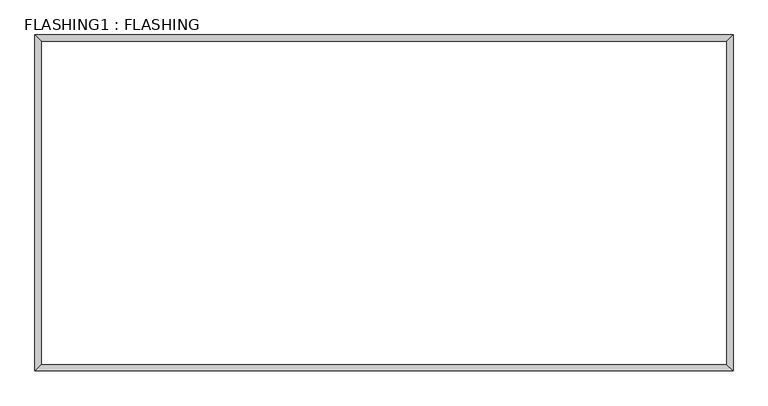
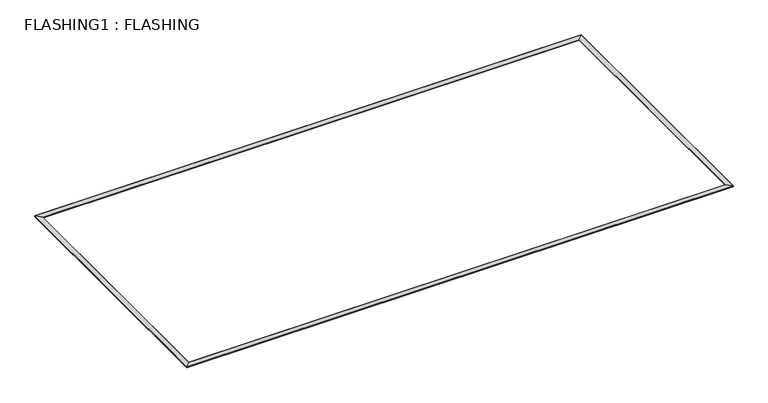
"""IFC4 building model written with IfcOpenShell, lengths in millimetres: proxy geometry, FLASHING1 : FLASHING."""

from ifc_helpers import new_model, si_unit, origin, place, context, project, spatial, faceted_brep, source, transform, mapped, element, save


def flashing1_flashing_4cce81cf(model_context):
    return source(origin(), model_context, "Body", "Brep", [
        faceted_brep([(40720.0, 40009.5208589, 18739.9720055), (40720.0, 40009.5208589, 18724.9720055), (40720.0, 19989.5208589, 18724.9720055), (40720.0, 19989.5208589, 18739.9720055), (40721.0, 40010.5208589, 18750.9720055), (40721.0, 40010.5208589, 18739.9720055), (40721.0, 19988.5208589, 18739.9720055), (40721.0, 19988.5208589, 18750.9720055), (40749.0, 40038.5208589, 18819.1280996), (40749.0, 40038.5208589, 18750.9720055), (40749.0, 19960.5208589, 18750.9720055), (40749.0, 19960.5208589, 18819.1280996), (40371.0, 39660.5208589, 18804.3045702), (40371.0, 20338.5208589, 18804.3045702), (40371.0, 39660.5208589, 18750.9720055), (40371.0, 20338.5208589, 18750.9720055), (40399.0, 39688.5208589, 18739.9720055), (40399.0, 39688.5208589, 18750.9720055), (40399.0, 20310.5208589, 18750.9720055), (40399.0, 20310.5208589, 18739.9720055), (40400.0, 39689.5208589, 18724.9720055), (40400.0, 39689.5208589, 18739.9720055), (40400.0, 20309.5208589, 18739.9720055), (40400.0, 20309.5208589, 18724.9720055), (40398.0, 39687.5208589, 18749.9720055), (40398.0, 39687.5208589, 18724.9720055), (40398.0, 20311.5208589, 18724.9720055), (40398.0, 20311.5208589, 18749.9720055), (40370.0, 39659.5208589, 18805.2661232), (40370.0, 39659.5208589, 18749.9720055), (40370.0, 20339.5208589, 18749.9720055), (40370.0, 20339.5208589, 18805.2661232), (40750.0, 40039.5208589, 18820.168084), (40750.0, 19959.5208589, 18820.168084), (40750.0, 40039.5208589, 18749.9720055), (40750.0, 19959.5208589, 18749.9720055), (40722.0, 40011.5208589, 18724.9720055), (40722.0, 40011.5208589, 18749.9720055), (40722.0, 19987.5208589, 18749.9720055), (40722.0, 19987.5208589, 18724.9720055), (-935.0, 19989.5208589, 18724.9720055), (-935.0, 19989.5208589, 18739.9720055), (-936.0, 19988.5208589, 18739.9720055), (-936.0, 19988.5208589, 18750.9720055), (-964.0, 19960.5208589, 18750.9720055), (-964.0, 19960.5208589, 18819.1280996), (-586.0, 20338.5208589, 18804.3045702), (-586.0, 20338.5208589, 18750.9720055), (-614.0, 20310.5208589, 18750.9720055), (-614.0, 20310.5208589, 18739.9720055), (-615.0, 20309.5208589, 18739.9720055), (-615.0, 20309.5208589, 18724.9720055), (-613.0, 20311.5208589, 18724.9720055), (-613.0, 20311.5208589, 18749.9720055), (-585.0, 20339.5208589, 18749.9720055), (-585.0, 20339.5208589, 18805.2661232), (-965.0, 19959.5208589, 18820.168084), (-965.0, 19959.5208589, 18749.9720055), (-937.0, 19987.5208589, 18749.9720055), (-937.0, 19987.5208589, 18724.9720055), (-935.0, 40009.5208589, 18724.9720055), (-935.0, 40009.5208589, 18739.9720055), (-936.0, 40010.5208589, 18739.9720055), (-936.0, 40010.5208589, 18750.9720055), (-964.0, 40038.5208589, 18750.9720055), (-964.0, 40038.5208589, 18819.1280996), (-586.0, 39660.5208589, 18804.3045702), (-586.0, 39660.5208589, 18750.9720055), (-614.0, 39688.5208589, 18750.9720055), (-614.0, 39688.5208589, 18739.9720055), (-615.0, 39689.5208589, 18739.9720055), (-615.0, 39689.5208589, 18724.9720055), (-613.0, 39687.5208589, 18724.9720055), (-613.0, 39687.5208589, 18749.9720055), (-585.0, 39659.5208589, 18749.9720055), (-585.0, 39659.5208589, 18805.2661232), (-965.0, 40039.5208589, 18820.168084), (-965.0, 40039.5208589, 18749.9720055), (-937.0, 40011.5208589, 18749.9720055), (-937.0, 40011.5208589, 18724.9720055)], [[[0, 1, 2, 3]], [[4, 5, 6, 7]], [[8, 9, 10, 11]], [[12, 8, 11, 13]], [[14, 12, 13, 15]], [[16, 17, 18, 19]], [[20, 21, 22, 23]], [[24, 25, 26, 27]], [[28, 29, 30, 31]], [[32, 28, 31, 33]], [[34, 32, 33, 35]], [[36, 37, 38, 39]], [[3, 2, 40, 41]], [[7, 6, 42, 43]], [[11, 10, 44, 45]], [[13, 11, 45, 46]], [[15, 13, 46, 47]], [[19, 18, 48, 49]], [[23, 22, 50, 51]], [[27, 26, 52, 53]], [[31, 30, 54, 55]], [[33, 31, 55, 56]], [[35, 33, 56, 57]], [[39, 38, 58, 59]], [[41, 40, 60, 61]], [[43, 42, 62, 63]], [[45, 44, 64, 65]], [[46, 45, 65, 66]], [[47, 46, 66, 67]], [[49, 48, 68, 69]], [[51, 50, 70, 71]], [[53, 52, 72, 73]], [[55, 54, 74, 75]], [[56, 55, 75, 76]], [[57, 56, 76, 77]], [[59, 58, 78, 79]], [[61, 60, 1, 0]], [[5, 62, 42, 6], [3, 41, 61, 0]], [[63, 62, 5, 4]], [[9, 64, 44, 10], [7, 43, 63, 4]], [[65, 64, 9, 8]], [[66, 65, 8, 12]], [[67, 66, 12, 14]], [[17, 68, 48, 18], [15, 47, 67, 14]], [[69, 68, 17, 16]], [[21, 70, 50, 22], [19, 49, 69, 16]], [[71, 70, 21, 20]], [[23, 51, 71, 20], [25, 72, 52, 26]], [[73, 72, 25, 24]], [[27, 53, 73, 24], [29, 74, 54, 30]], [[75, 74, 29, 28]], [[76, 75, 28, 32]], [[77, 76, 32, 34]], [[35, 57, 77, 34], [37, 78, 58, 38]], [[79, 78, 37, 36]], [[39, 59, 79, 36], [1, 60, 40, 2]]]),
    ])


if __name__ == "__main__":
    model = new_model("IFC4")
    model_context = context("Model", 3, world=origin())
    ifc_project = project(units=[si_unit("LENGTHUNIT", "METRE", prefix="MILLI")], contexts=[model_context])
    site = spatial("IfcSite", under=ifc_project)
    building = spatial("IfcBuilding", under=site)
    placement = place(None, origin())
    flashing1_flashing_shape = flashing1_flashing_4cce81cf(model_context)
    element("IfcBuildingElementProxy", 1, Name="FLASHING1 : FLASHING", ObjectType="FLASHING1 : FLASHING", at=placement, inside=building, context=model_context, shape_type="MappedRepresentation", body=[
        mapped(flashing1_flashing_shape, transform((0.0, 0.0, 0.0), x_axis=(1.0, 0.0, 0.0), y_axis=(0.0, 1.0, 0.0), z_axis=(0.0, 0.0, 1.0))),
    ])
    save(model, "model.ifc")
